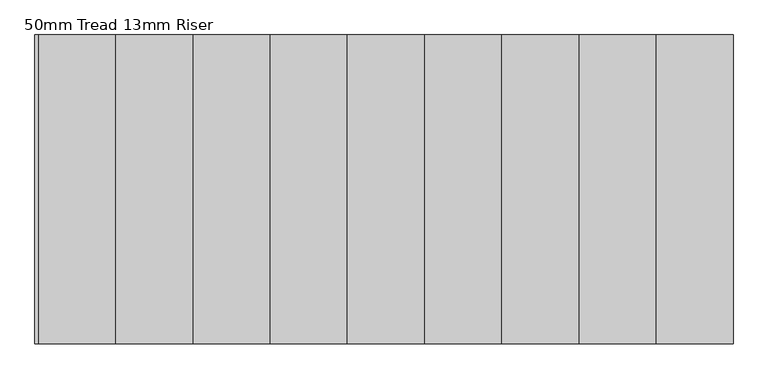
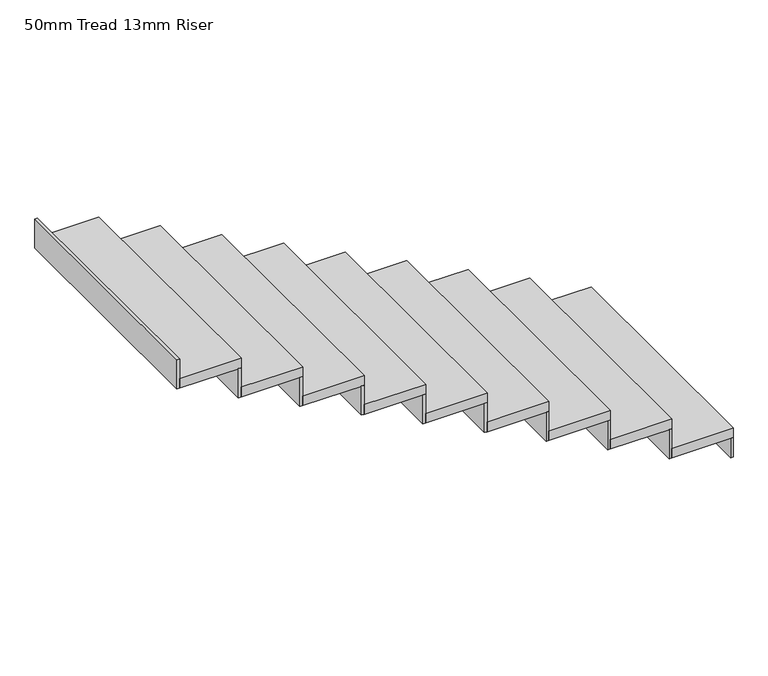
"""IFC4 building model written with IfcOpenShell, lengths in millimetres: stair flight geometry, 50mm Tread 13mm Riser."""

from ifc_helpers import new_model, si_unit, frame, origin, origin_with_axes, place, context, project, spatial, polyline, outline, extrude, source, transform, mapped, element, save


def stair_flight_50mm_tread_13mm_riser_f6205c5f(model_context):
    return source(origin(), model_context, "Body", "SweptSolid", [
        extrude(outline(polyline([(22383.7289955, -4912.5395691), (22396.2289955, -4912.5395691), (22396.2289955, -6112.5395691), (22383.7289955, -6112.5395691), (22383.7289955, -4912.5395691)])), origin_with_axes(), (0.0, 0.0, 1.0), 100.0),
        extrude(outline(polyline([(22096.2289955, -6112.5395691), (22096.2289955, -4912.5395691), (22396.2289955, -4912.5395691), (22396.2289955, -6112.5395691), (22096.2289955, -6112.5395691)])), frame((0.0, 0.0, 100.0), z_axis=(0.0, 0.0, 1.0), x_axis=(1.0, 0.0, 0.0)), (0.0, 0.0, 1.0), 50.0),
        extrude(outline(polyline([(22083.7289955, -4912.5395691), (22096.2289955, -4912.5395691), (22096.2289955, -6112.5395691), (22083.7289955, -6112.5395691), (22083.7289955, -4912.5395691)])), frame((0.0, 0.0, 100.0), z_axis=(0.0, 0.0, 1.0), x_axis=(1.0, 0.0, 0.0)), (0.0, 0.0, 1.0), 150.0),
        extrude(outline(polyline([(21796.2289955, -6112.5395691), (21796.2289955, -4912.5395691), (22096.2289955, -4912.5395691), (22096.2289955, -6112.5395691), (21796.2289955, -6112.5395691)])), frame((0.0, 0.0, 250.0), z_axis=(0.0, 0.0, 1.0), x_axis=(1.0, 0.0, 0.0)), (0.0, 0.0, 1.0), 50.0),
        extrude(outline(polyline([(21783.7289955, -4912.5395691), (21796.2289955, -4912.5395691), (21796.2289955, -6112.5395691), (21783.7289955, -6112.5395691), (21783.7289955, -4912.5395691)])), frame((0.0, 0.0, 250.0), z_axis=(0.0, 0.0, 1.0), x_axis=(1.0, 0.0, 0.0)), (0.0, 0.0, 1.0), 150.0),
        extrude(outline(polyline([(21496.2289955, -6112.5395691), (21496.2289955, -4912.5395691), (21796.2289955, -4912.5395691), (21796.2289955, -6112.5395691), (21496.2289955, -6112.5395691)])), frame((0.0, 0.0, 400.0), z_axis=(0.0, 0.0, 1.0), x_axis=(1.0, 0.0, 0.0)), (0.0, 0.0, 1.0), 50.0),
        extrude(outline(polyline([(21483.7289955, -4912.5395691), (21496.2289955, -4912.5395691), (21496.2289955, -6112.5395691), (21483.7289955, -6112.5395691), (21483.7289955, -4912.5395691)])), frame((0.0, 0.0, 400.0), z_axis=(0.0, 0.0, 1.0), x_axis=(1.0, 0.0, 0.0)), (0.0, 0.0, 1.0), 150.0),
        extrude(outline(polyline([(21196.2289955, -6112.5395691), (21196.2289955, -4912.5395691), (21496.2289955, -4912.5395691), (21496.2289955, -6112.5395691), (21196.2289955, -6112.5395691)])), frame((0.0, 0.0, 550.0), z_axis=(0.0, 0.0, 1.0), x_axis=(1.0, 0.0, 0.0)), (0.0, 0.0, 1.0), 50.0),
        extrude(outline(polyline([(21183.7289955, -4912.5395691), (21196.2289955, -4912.5395691), (21196.2289955, -6112.5395691), (21183.7289955, -6112.5395691), (21183.7289955, -4912.5395691)])), frame((0.0, 0.0, 550.0), z_axis=(0.0, 0.0, 1.0), x_axis=(1.0, 0.0, 0.0)), (0.0, 0.0, 1.0), 150.0),
        extrude(outline(polyline([(20896.2289955, -6112.5395691), (20896.2289955, -4912.5395691), (21196.2289955, -4912.5395691), (21196.2289955, -6112.5395691), (20896.2289955, -6112.5395691)])), frame((0.0, 0.0, 700.0), z_axis=(0.0, 0.0, 1.0), x_axis=(1.0, 0.0, 0.0)), (0.0, 0.0, 1.0), 50.0),
        extrude(outline(polyline([(20883.7289955, -4912.5395691), (20896.2289955, -4912.5395691), (20896.2289955, -6112.5395691), (20883.7289955, -6112.5395691), (20883.7289955, -4912.5395691)])), frame((0.0, 0.0, 700.0), z_axis=(0.0, 0.0, 1.0), x_axis=(1.0, 0.0, 0.0)), (0.0, 0.0, 1.0), 150.0),
        extrude(outline(polyline([(20596.2289955, -6112.5395691), (20596.2289955, -4912.5395691), (20896.2289955, -4912.5395691), (20896.2289955, -6112.5395691), (20596.2289955, -6112.5395691)])), frame((0.0, 0.0, 850.0), z_axis=(0.0, 0.0, 1.0), x_axis=(1.0, 0.0, 0.0)), (0.0, 0.0, 1.0), 50.0),
        extrude(outline(polyline([(20583.7289955, -4912.5395691), (20596.2289955, -4912.5395691), (20596.2289955, -6112.5395691), (20583.7289955, -6112.5395691), (20583.7289955, -4912.5395691)])), frame((0.0, 0.0, 850.0), z_axis=(0.0, 0.0, 1.0), x_axis=(1.0, 0.0, 0.0)), (0.0, 0.0, 1.0), 150.0),
        extrude(outline(polyline([(20296.2289955, -6112.5395691), (20296.2289955, -4912.5395691), (20596.2289955, -4912.5395691), (20596.2289955, -6112.5395691), (20296.2289955, -6112.5395691)])), frame((0.0, 0.0, 1000.0), z_axis=(0.0, 0.0, 1.0), x_axis=(1.0, 0.0, 0.0)), (0.0, 0.0, 1.0), 50.0),
        extrude(outline(polyline([(20283.7289955, -4912.5395691), (20296.2289955, -4912.5395691), (20296.2289955, -6112.5395691), (20283.7289955, -6112.5395691), (20283.7289955, -4912.5395691)])), frame((0.0, 0.0, 1000.0), z_axis=(0.0, 0.0, 1.0), x_axis=(1.0, 0.0, 0.0)), (0.0, 0.0, 1.0), 150.0),
        extrude(outline(polyline([(19996.2289955, -6112.5395691), (19996.2289955, -4912.5395691), (20296.2289955, -4912.5395691), (20296.2289955, -6112.5395691), (19996.2289955, -6112.5395691)])), frame((0.0, 0.0, 1150.0), z_axis=(0.0, 0.0, 1.0), x_axis=(1.0, 0.0, 0.0)), (0.0, 0.0, 1.0), 50.0),
        extrude(outline(polyline([(19983.7289955, -4912.5395691), (19996.2289955, -4912.5395691), (19996.2289955, -6112.5395691), (19983.7289955, -6112.5395691), (19983.7289955, -4912.5395691)])), frame((0.0, 0.0, 1150.0), z_axis=(0.0, 0.0, 1.0), x_axis=(1.0, 0.0, 0.0)), (0.0, 0.0, 1.0), 150.0),
        extrude(outline(polyline([(19683.7289955, -4912.5395691), (19696.2289955, -4912.5395691), (19696.2289955, -6112.5395691), (19683.7289955, -6112.5395691), (19683.7289955, -4912.5395691)])), frame((0.0, 0.0, 1300.0), z_axis=(0.0, 0.0, 1.0), x_axis=(1.0, 0.0, 0.0)), (0.0, 0.0, 1.0), 150.0),
        extrude(outline(polyline([(19696.2289955, -6112.5395691), (19696.2289955, -4912.5395691), (19996.2289955, -4912.5395691), (19996.2289955, -6112.5395691), (19696.2289955, -6112.5395691)])), frame((0.0, 0.0, 1300.0), z_axis=(0.0, 0.0, 1.0), x_axis=(1.0, 0.0, 0.0)), (0.0, 0.0, 1.0), 50.0),
    ])


if __name__ == "__main__":
    model = new_model("IFC4")
    model_context = context("Model", 3, world=origin())
    ifc_project = project(units=[si_unit("LENGTHUNIT", "METRE", prefix="MILLI")], contexts=[model_context])
    site = spatial("IfcSite", under=ifc_project)
    building = spatial("IfcBuilding", under=site)
    placement = place(None, origin())
    stair_flight_50mm_tread_13mm_riser_shape = stair_flight_50mm_tread_13mm_riser_f6205c5f(model_context)
    element("IfcStairFlight", 1, ObjectType="50mm Tread 13mm Riser", at=placement, inside=building, context=model_context, shape_type="MappedRepresentation", body=[
        mapped(stair_flight_50mm_tread_13mm_riser_shape, transform((0.0, 0.0, 0.0), x_axis=(1.0, 0.0, 0.0), y_axis=(0.0, 1.0, 0.0), z_axis=(0.0, 0.0, 1.0))),
    ])
    save(model, "model.ifc")
